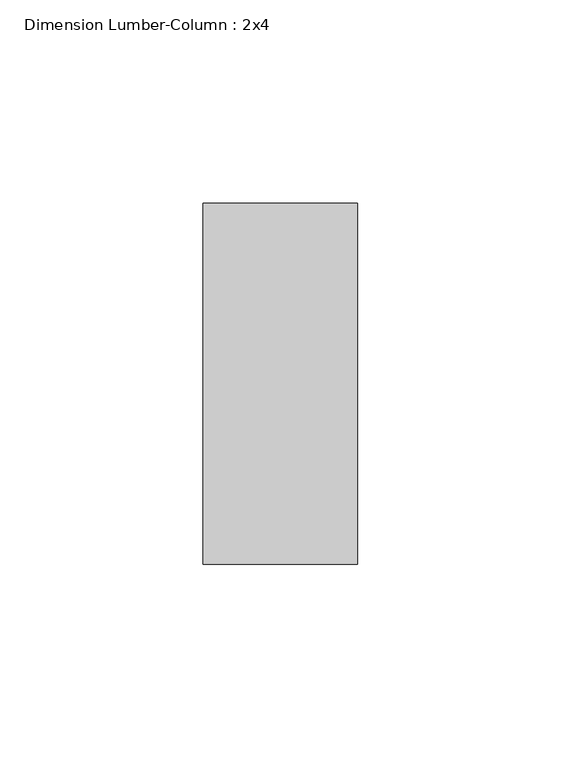
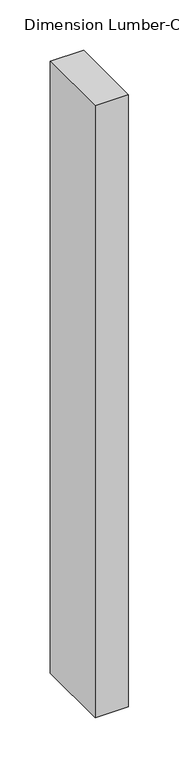
"""IFC4 building model written with IfcOpenShell, lengths in millimetres: column geometry, Dimension Lumber-Column : 2x4."""

from ifc_helpers import new_model, si_unit, frame, origin, place, context, project, spatial, polyline, outline, extrude, source, transform, mapped, element, save


def dimension_lumber_column_2x4_b47e0866(model_context):
    return source(origin(), model_context, "Body", "SweptSolid", [
        extrude(outline(polyline([(19.05, -44.45), (-19.05, -44.45), (-19.05, 44.45), (19.05, 44.45), (19.05, -44.45)])), frame((0.0, 0.0, 56.35625), z_axis=(0.0, 0.0, 1.0), x_axis=(1.0, 0.0, 0.0)), (0.0, 0.0, 1.0), 742.553125),
    ])


if __name__ == "__main__":
    model = new_model("IFC4")
    model_context = context("Model", 3, world=origin())
    ifc_project = project(units=[si_unit("LENGTHUNIT", "METRE", prefix="MILLI")], contexts=[model_context])
    site = spatial("IfcSite", under=ifc_project)
    building = spatial("IfcBuilding", under=site)
    placement = place(None, origin())
    dimension_lumber_column_2x4_shape = dimension_lumber_column_2x4_b47e0866(model_context)
    element("IfcColumn", 1, ObjectType="Dimension Lumber-Column : 2x4", at=placement, inside=building, context=model_context, shape_type="MappedRepresentation", body=[
        mapped(dimension_lumber_column_2x4_shape, transform((0.0, 0.0, 0.0), x_axis=(1.0, 0.0, 0.0), y_axis=(0.0, 1.0, 0.0), z_axis=(0.0, 0.0, 1.0))),
    ])
    save(model, "model.ifc")

# Revit data of these elements
# Type "Dimension Lumber-Column : 2x4"
#   Int Type = "Interior"
#   Assembly Code = "B10"
#   Cost = 8.05
#   A = 0.0364583 SF
#   b = 0' - 1 1/2"
#   d = 0' - 3 1/2"
#   Structural Material [instance default] = Softwood, Lumber
# Element 1 (IfcColumn, "Dimension Lumber-Column : 2x4")
#   Structural Material = Douglas Fir #2
#   Materials on its faces: "Douglas Fir #2"
# Materials
#   "Softwood, Lumber": class "Wood", colour RGB 223 192 134, transparency 0, Description = "Pinus Echinata", Cost = 0
#   "Douglas Fir #2": class "Wood", colour RGB 223 192 134, transparency 0, Description = "Pinus Echinata", Cost = 0
